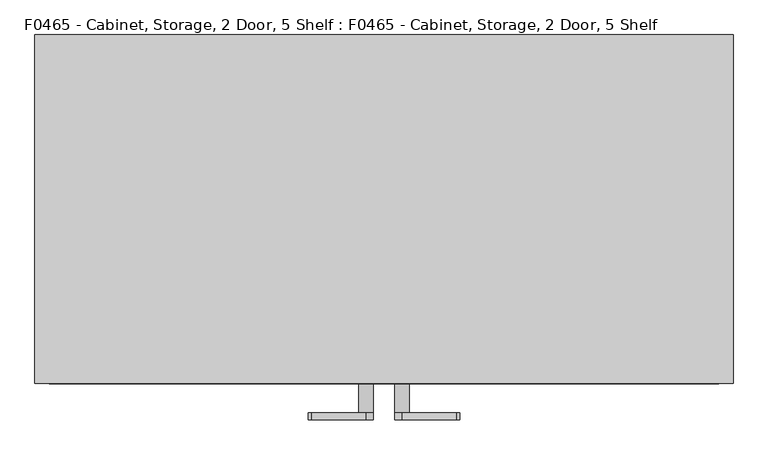
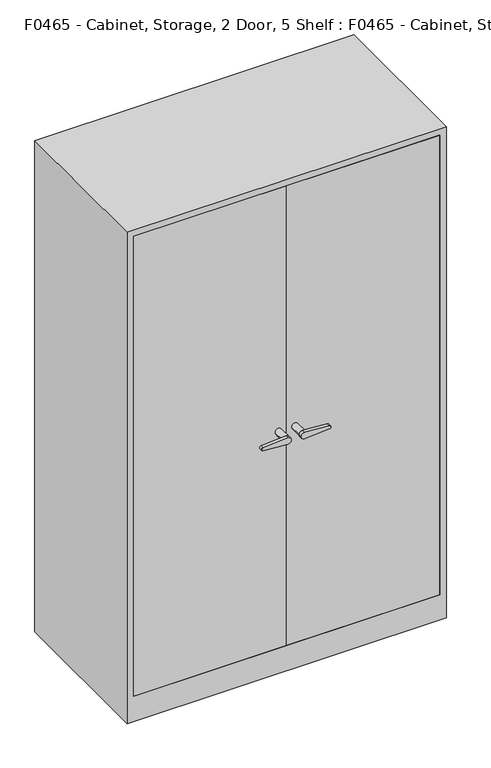
"""IFC4 building model written with IfcOpenShell, lengths in millimetres: proxy geometry, F0465 - Cabinet, Storage, 2 Door, 5 Shelf : F0465 - Cabinet, Storage, 2 Door, 5 Shelf."""

from ifc_helpers import new_model, si_unit, point, frame, frame_2d, origin, origin_with_axes, place, context, project, spatial, polyline, circle_curve, trimmed, segment, composite_curve, outline, extrude, faceted_brep, source, transform, mapped, element, save


def f0465_cabinet_storage_2_door_5_shelf_f0465_cabinet_storage_2_be5e22c5(model_context):
    return source(origin(), model_context, "Body", "SolidModel", [
        extrude(outline(composite_curve([segment(trimmed(circle_curve(frame_2d((975.7942264, -31.5214938)), 12.7), [point((963.0942264, -31.5214938))], [point((988.4942264, -31.5214938))], False, "CARTESIAN"), True, "CONTINUOUS"), segment(polyline([(988.4942264, -31.5214938), (981.8203114, -126.9629251)]), True, "CONTINUOUS"), segment(trimmed(circle_curve(frame_2d((975.7942264, -126.1160141)), 6.0853068), [point((981.8203114, -126.9629251))], [point((969.7681414, -126.9629251))], False, "CARTESIAN"), True, "CONTINUOUS"), segment(polyline([(969.7681414, -126.9629251), (963.0942264, -31.5214938)]), True, "CONTINUOUS")], self_intersect=False)), frame((0.0, -368.3, 0.0), z_axis=(0.0, 1.0, 0.0), x_axis=(0.0, 0.0, 1.0)), (0.0, 0.0, 1.0), 12.7),
        extrude(outline(composite_curve([segment(trimmed(circle_curve(frame_2d((975.7942264, -31.5214938)), 12.7), [point((975.7942264, -18.8214938))], [point((975.7942264, -44.2214938))], False, "CARTESIAN"), True, "CONTINUOUS"), segment(trimmed(circle_curve(frame_2d((975.7942264, -31.5214938)), 12.7), [point((975.7942264, -44.2214938))], [point((975.7942264, -18.8214938))], False, "CARTESIAN"), True, "CONTINUOUS")], self_intersect=False)), frame((0.0, -355.6, 0.0), z_axis=(0.0, 1.0, 0.0), x_axis=(0.0, 0.0, 1.0)), (0.0, 0.0, 1.0), 50.8),
        extrude(outline(composite_curve([segment(polyline([(963.0942264, 31.5214938), (969.7681414, 126.9629251)]), True, "CONTINUOUS"), segment(trimmed(circle_curve(frame_2d((975.7942264, 126.1160141)), 6.0853068), [point((969.7681414, 126.9629251))], [point((981.8203114, 126.9629251))], False, "CARTESIAN"), True, "CONTINUOUS"), segment(polyline([(981.8203114, 126.9629251), (988.4942264, 31.5214938)]), True, "CONTINUOUS"), segment(trimmed(circle_curve(frame_2d((975.7942264, 31.5214938)), 12.7), [point((988.4942264, 31.5214938))], [point((963.0942264, 31.5214938))], False, "CARTESIAN"), True, "CONTINUOUS")], self_intersect=False)), frame((0.0, -368.3, 0.0), z_axis=(0.0, 1.0, 0.0), x_axis=(0.0, 0.0, 1.0)), (0.0, 0.0, 1.0), 12.7),
        extrude(outline(composite_curve([segment(trimmed(circle_curve(frame_2d((975.7942264, 31.5214938)), 12.7), [point((975.7942264, 18.8214938))], [point((975.7942264, 44.2214938))], False, "CARTESIAN"), True, "CONTINUOUS"), segment(trimmed(circle_curve(frame_2d((975.7942264, 31.5214938)), 12.7), [point((975.7942264, 44.2214938))], [point((975.7942264, 18.8214938))], False, "CARTESIAN"), True, "CONTINUOUS")], self_intersect=False)), frame((0.0, -355.6, 0.0), z_axis=(0.0, 1.0, 0.0), x_axis=(0.0, 0.0, 1.0)), (0.0, 0.0, 1.0), 50.8),
        extrude(outline(polyline([(0.0, -304.8), (0.0, -279.4), (584.2, -279.4), (584.2, -304.8), (0.0, -304.8)])), frame((0.0, 0.0, 101.6), z_axis=(0.0, 0.0, 1.0), x_axis=(1.0, 0.0, 0.0)), (0.0, 0.0, 1.0), 1854.2),
        extrude(outline(polyline([(0.0, -304.8), (-584.2, -304.8), (-584.2, -279.4), (0.0, -279.4), (0.0, -304.8)])), frame((0.0, 0.0, 101.6), z_axis=(0.0, 0.0, 1.0), x_axis=(1.0, 0.0, 0.0)), (0.0, 0.0, 1.0), 1854.2),
        faceted_brep([(609.6, -304.8, 1981.2), (-609.6, -304.8, 1981.2), (-609.6, -304.8, 0.0), (609.6, -304.8, 0.0), (-584.2, -304.8, 1955.8), (584.2, -304.8, 1955.8), (584.2, -304.8, 101.6), (-584.2, -304.8, 101.6), (609.6, 304.8, 1981.2), (-609.6, 304.8, 1981.2), (-609.6, 304.8, 0.0), (609.6, 304.8, 0.0), (-584.2, 279.4, 1955.8), (584.2, 279.4, 1955.8), (584.2, 279.4, 101.6), (-584.2, 279.4, 101.6)], [[[0, 1, 2, 3], [4, 5, 6, 7]], [[1, 0, 8, 9]], [[2, 1, 9, 10]], [[3, 2, 10, 11]], [[8, 0, 3, 11]], [[5, 4, 12, 13]], [[6, 5, 13, 14]], [[7, 6, 14, 15]], [[4, 7, 15, 12]], [[9, 8, 11, 10]], [[13, 12, 15, 14]]]),
        extrude(outline(polyline([(-609.6, 304.8), (609.6, 304.8), (609.6, -304.8), (-609.6, -304.8), (-609.6, 0.0), (-609.6, 304.8)])), origin_with_axes(), (0.0, 0.0, 1.0), 1981.2),
    ])


if __name__ == "__main__":
    model = new_model("IFC4")
    model_context = context("Model", 3, world=origin())
    ifc_project = project(units=[si_unit("LENGTHUNIT", "METRE", prefix="MILLI")], contexts=[model_context])
    site = spatial("IfcSite", under=ifc_project)
    building = spatial("IfcBuilding", under=site)
    placement = place(None, origin())
    f0465_cabinet_storage_2_door_5_shelf_f0465_cabinet_storage_2_shape = f0465_cabinet_storage_2_door_5_shelf_f0465_cabinet_storage_2_be5e22c5(model_context)
    element("IfcBuildingElementProxy", 1, Name="F0465 - Cabinet, Storage, 2 Door, 5 Shelf : F0465 - Cabinet, Storage, 2 Door, 5 Shelf", ObjectType="F0465 - Cabinet, Storage, 2 Door, 5 Shelf : F0465 - Cabinet, Storage, 2 Door, 5 Shelf", at=placement, inside=building, context=model_context, shape_type="MappedRepresentation", body=[
        mapped(f0465_cabinet_storage_2_door_5_shelf_f0465_cabinet_storage_2_shape, transform((0.0, 0.0, 0.0), x_axis=(1.0, 0.0, 0.0), y_axis=(0.0, 1.0, 0.0), z_axis=(0.0, 0.0, 1.0))),
    ])
    save(model, "model.ifc")

# Revit data of these elements
# Project information
#   Room Abbreviation = "VXER1"
#   Room Description = "XRay, Veterinary (VXER1)"
#   Sheets - Total = "5"
#   Project Issue Date = "Issue Date"
#   Project Status = "Project Status"
#   Client Name = "Owner"
#   Project Address = "Enter address here"
#   Project Name = "Project Name"
#   Project Number = "Project Number"
#   Publication Date = "30-Jan-15"
# Type "F0465 - Cabinet, Storage, 2 Door, 5 Shelf : F0465 - Cabinet, Storage, 2 Door, 5 Shelf"
#   Watts2 = "0"
#   Watts1 = "0"
#   Unit_Issue = "EA"
#   UTIL_6_Misc = "-"
#   UTIL_5_NonMedGas = "-"
#   UTIL_4_MiscGas = "-"
#   UTIL_3_MedGas = "-"
#   UTIL_2_Elec = "-"
#   UTIL_1_WaterDrain = "-"
#   Nomenclature = "Cabinet, Storage, 2 Door, 5 Shelf"
#   NSN = "7100"
#   Location [instance default] = ""
#   JSN = "F0465"
#   Fund_Source_VA = "-"
#   Fund_Source_Navy = "-"
#   Fund_Source_Army = "-"
#   Fund_Source_AF = "-"
#   ELEC_Volts2 = "0"
#   ELEC_Volts1 = "0"
#   ELEC_Phase2 = "0"
#   ELEC_Phase1 = "0"
#   ELEC_HertzSwitch = "0"
#   ELEC_HertzDependent = "0"
#   ELEC_Hertz = "0"
#   ELEC_Amps2 = "0"
#   ELEC_Amps1 = "0"
#   DetailDescription = "Storage cabinet, 78\" high X 48\" wide X 24\" deep with two (2) doors and five (5) adjustable shelves."
#   CAT_VA = "C"
#   CAT_Navy = "C"
#   CAT_IHS = "-"
#   CAT_Army = "C"
#   CAT_AF = "C"
#   BTUperhour = "0"
#   Weight_IP = 233
#   DIM_Width_IP = 4' - 0"
#   DIM_Height_IP = 6' - 6"
#   DIM_Depth_IP = 2' - 0"
# Element 1 (IfcBuildingElementProxy, "F0465 - Cabinet, Storage, 2 Door, 5 Shelf : F0465 - Cabinet, Storage, 2 Door, 5 Shelf")
#   Materials on its faces: "EquipSpace"
# Materials
#   "EquipSpace": class "Unassigned", colour RGB 221 217 195, transparency 0.5
